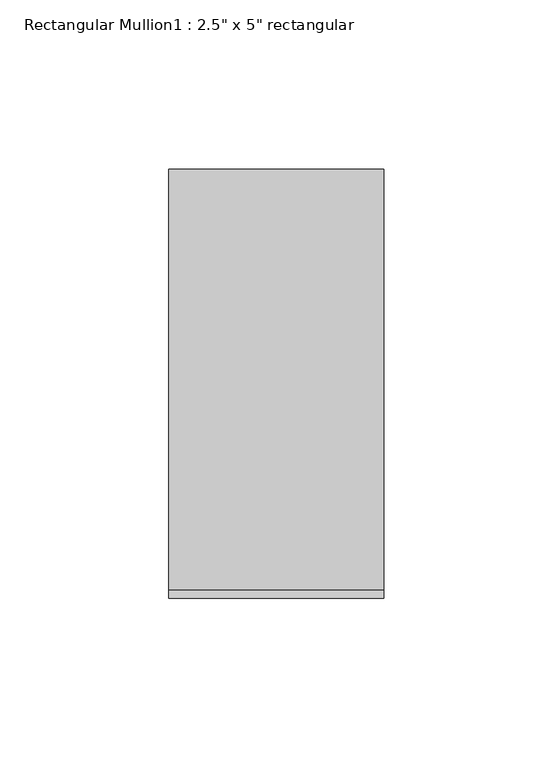
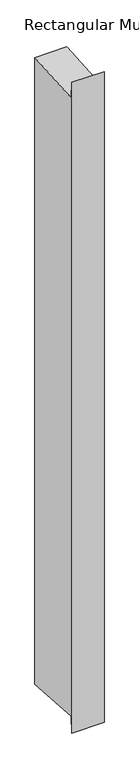
"""IFC4 building model written with IfcOpenShell, lengths in millimetres: member geometry."""

from ifc_helpers import new_model, si_unit, frame, origin, place, context, project, spatial, polyline, outline, extrude, source, transform, mapped, element, save


def member_7395c1fc(model_context):
    return source(origin(), model_context, "Body", "SweptSolid", [
        extrude(outline(polyline([(-63.5, 29.5074223), (-61.1020145, -4.4004678), (63.5, 4.4114583), (63.5, -1307.1798222), (-61.1020145, -1298.3678961), (-63.5, -1332.2757861), (-63.5, 29.5074223)])), frame((-63.5, 0.0, 0.0), z_axis=(1.0, 0.0, 0.0), x_axis=(0.0, 1.0, 0.0)), (0.0, 0.0, 1.0), 63.5),
    ])


if __name__ == "__main__":
    model = new_model("IFC4")
    model_context = context("Model", 3, world=origin())
    ifc_project = project(units=[si_unit("LENGTHUNIT", "METRE", prefix="MILLI")], contexts=[model_context])
    site = spatial("IfcSite", under=ifc_project)
    building = spatial("IfcBuilding", under=site)
    placement = place(None, origin())
    member_shape = member_7395c1fc(model_context)
    element("IfcMember", 1, ObjectType="Rectangular Mullion1 : 2.5\" x 5\" rectangular", at=placement, inside=building, context=model_context, shape_type="MappedRepresentation", body=[
        mapped(member_shape, transform((0.0, 0.0, 0.0), x_axis=(1.0, 0.0, 0.0), y_axis=(0.0, 1.0, 0.0), z_axis=(0.0, 0.0, 1.0))),
    ])
    save(model, "model.ifc")

# Revit data of these elements
# Type "Rectangular Mullion1 : 2.5\" x 5\" rectangular"
#   built-in parameter 1007304 = 0.416667 (stored number, unit not read)
#   built-in parameter 1007301 = 0.104167 (stored number, unit not read)
#   built-in parameter 1007300 = 0.104167 (stored number, unit not read)
# Element 1 (IfcMember, "Rectangular Mullion1 : 2.5\" x 5\" rectangular")
#   Materials on its faces: "support-frame"
# Materials
#   "support-frame": class "Unassigned", colour RGB 233 233 233, transparency 0, Cost = 0
